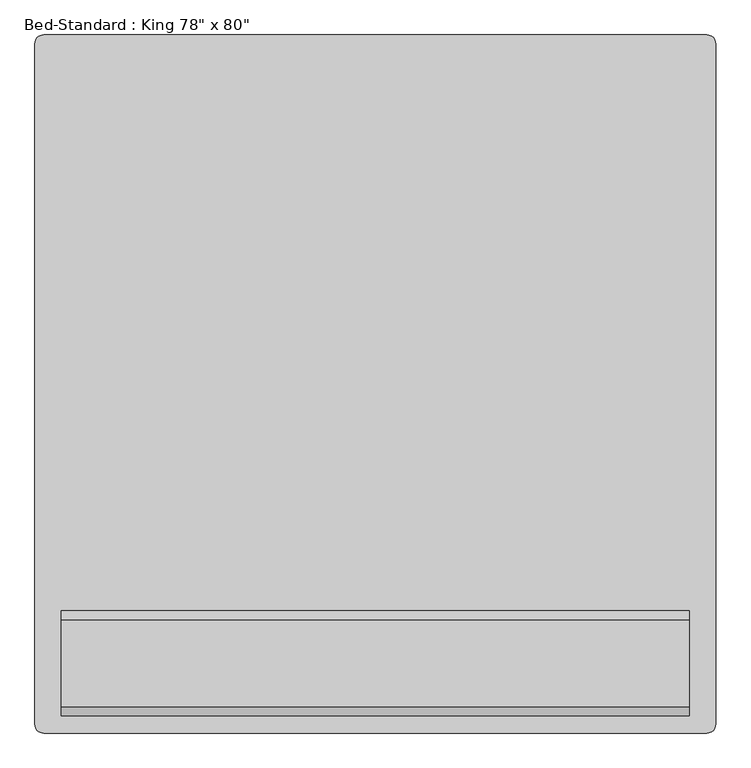
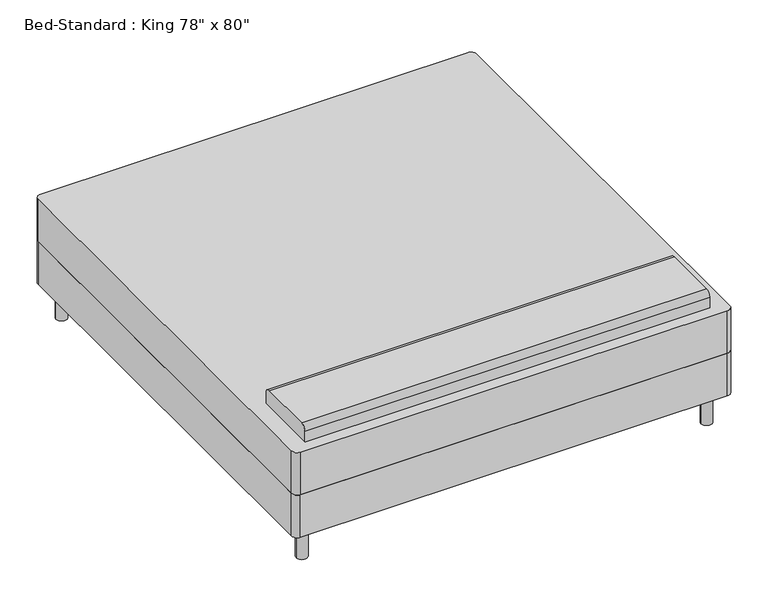
"""IFC4 building model written with IfcOpenShell, lengths in millimetres: furniture geometry."""

from ifc_helpers import new_model, si_unit, point, frame, frame_2d, origin, origin_with_axes, place, context, project, spatial, polyline, circle_curve, trimmed, segment, composite_curve, outline, extrude, source, transform, mapped, element, save


def furniture_df776289(model_context):
    return source(origin(), model_context, "Body", "SweptSolid", [
        extrude(outline(composite_curve([segment(trimmed(circle_curve(frame_2d((-693.7114754, 1036.195082)), 25.4), [point((-719.1114754, 1036.195082))], [point((-693.7114754, 1061.595082))], False, "CARTESIAN"), True, "CONTINUOUS"), segment(polyline([(-693.7114754, 1061.595082), (1236.6885246, 1061.595082)]), True, "CONTINUOUS"), segment(trimmed(circle_curve(frame_2d((1236.6885246, 1036.195082)), 25.4), [point((1236.6885246, 1061.595082))], [point((1262.0885246, 1036.195082))], False, "CARTESIAN"), True, "CONTINUOUS"), segment(polyline([(1262.0885246, 1036.195082), (1262.0885246, -945.004918)]), True, "CONTINUOUS"), segment(trimmed(circle_curve(frame_2d((1236.6885246, -945.004918)), 25.4), [point((1262.0885246, -945.004918))], [point((1236.6885246, -970.404918))], False, "CARTESIAN"), True, "CONTINUOUS"), segment(polyline([(1236.6885246, -970.404918), (-693.7114754, -970.404918)]), True, "CONTINUOUS"), segment(trimmed(circle_curve(frame_2d((-693.7114754, -945.004918)), 25.4), [point((-693.7114754, -970.404918))], [point((-719.1114754, -945.004918))], False, "CARTESIAN"), True, "CONTINUOUS"), segment(polyline([(-719.1114754, -945.004918), (-719.1114754, 1036.195082)]), True, "CONTINUOUS")], self_intersect=False)), frame((0.0, 0.0, 152.4), z_axis=(0.0, 0.0, 1.0), x_axis=(1.0, 0.0, 0.0)), (0.0, 0.0, 1.0), 203.2),
        extrude(outline(composite_curve([segment(polyline([(-614.804918, 558.8), (-919.604918, 558.8), (-919.604918, 609.6)]), True, "CONTINUOUS"), segment(trimmed(circle_curve(frame_2d((-894.204918, 609.6)), 25.4), [point((-919.604918, 609.6))], [point((-894.204918, 635.0))], False, "CARTESIAN"), True, "CONTINUOUS"), segment(polyline([(-894.204918, 635.0), (-640.204918, 635.0)]), True, "CONTINUOUS"), segment(trimmed(circle_curve(frame_2d((-640.204918, 609.6)), 25.4), [point((-640.204918, 635.0))], [point((-614.804918, 609.6))], False, "CARTESIAN"), True, "CONTINUOUS"), segment(polyline([(-614.804918, 609.6), (-614.804918, 558.8)]), True, "CONTINUOUS")], self_intersect=False)), frame((-642.9114754, 0.0, 0.0), z_axis=(1.0, 0.0, 0.0), x_axis=(0.0, 1.0, 0.0)), (0.0, 0.0, 1.0), 1828.8),
        extrude(outline(composite_curve([segment(trimmed(circle_curve(frame_2d((-642.9114754, -894.204918)), 25.4), [point((-668.3114754, -894.204918))], [point((-617.5114754, -894.204918))], False, "CARTESIAN"), True, "CONTINUOUS"), segment(trimmed(circle_curve(frame_2d((-642.9114754, -894.204918)), 25.4), [point((-617.5114754, -894.204918))], [point((-668.3114754, -894.204918))], False, "CARTESIAN"), True, "CONTINUOUS")], self_intersect=False)), origin_with_axes(), (0.0, 0.0, 1.0), 152.4),
        extrude(outline(composite_curve([segment(trimmed(circle_curve(frame_2d((1185.8885246, -894.204918)), 25.4), [point((1160.4885246, -894.204918))], [point((1211.2885246, -894.204918))], False, "CARTESIAN"), True, "CONTINUOUS"), segment(trimmed(circle_curve(frame_2d((1185.8885246, -894.204918)), 25.4), [point((1211.2885246, -894.204918))], [point((1160.4885246, -894.204918))], False, "CARTESIAN"), True, "CONTINUOUS")], self_intersect=False)), origin_with_axes(), (0.0, 0.0, 1.0), 152.4),
        extrude(outline(composite_curve([segment(trimmed(circle_curve(frame_2d((1185.8885246, 985.395082)), 25.4), [point((1160.4885246, 985.395082))], [point((1211.2885246, 985.395082))], False, "CARTESIAN"), True, "CONTINUOUS"), segment(trimmed(circle_curve(frame_2d((1185.8885246, 985.395082)), 25.4), [point((1211.2885246, 985.395082))], [point((1160.4885246, 985.395082))], False, "CARTESIAN"), True, "CONTINUOUS")], self_intersect=False)), origin_with_axes(), (0.0, 0.0, 1.0), 152.4),
        extrude(outline(composite_curve([segment(trimmed(circle_curve(frame_2d((-642.9114754, 985.395082)), 25.4), [point((-668.3114754, 985.395082))], [point((-617.5114754, 985.395082))], False, "CARTESIAN"), True, "CONTINUOUS"), segment(trimmed(circle_curve(frame_2d((-642.9114754, 985.395082)), 25.4), [point((-617.5114754, 985.395082))], [point((-668.3114754, 985.395082))], False, "CARTESIAN"), True, "CONTINUOUS")], self_intersect=False)), origin_with_axes(), (0.0, 0.0, 1.0), 152.4),
        extrude(outline(composite_curve([segment(trimmed(circle_curve(frame_2d((-693.7114754, -945.004918)), 25.4), [point((-693.7114754, -970.404918))], [point((-719.1114754, -945.004918))], False, "CARTESIAN"), True, "CONTINUOUS"), segment(polyline([(-719.1114754, -945.004918), (-719.1114754, 1036.195082)]), True, "CONTINUOUS"), segment(trimmed(circle_curve(frame_2d((-693.7114754, 1036.195082)), 25.4), [point((-719.1114754, 1036.195082))], [point((-693.7114754, 1061.595082))], False, "CARTESIAN"), True, "CONTINUOUS"), segment(polyline([(-693.7114754, 1061.595082), (1236.6885246, 1061.595082)]), True, "CONTINUOUS"), segment(trimmed(circle_curve(frame_2d((1236.6885246, 1036.195082)), 25.4), [point((1236.6885246, 1061.595082))], [point((1262.0885246, 1036.195082))], False, "CARTESIAN"), True, "CONTINUOUS"), segment(polyline([(1262.0885246, 1036.195082), (1262.0885246, -945.004918)]), True, "CONTINUOUS"), segment(trimmed(circle_curve(frame_2d((1236.6885246, -945.004918)), 25.4), [point((1262.0885246, -945.004918))], [point((1236.6885246, -970.404918))], False, "CARTESIAN"), True, "CONTINUOUS"), segment(polyline([(1236.6885246, -970.404918), (-693.7114754, -970.404918)]), True, "CONTINUOUS")], self_intersect=False)), frame((0.0, 0.0, 355.6), z_axis=(0.0, 0.0, 1.0), x_axis=(1.0, 0.0, 0.0)), (0.0, 0.0, 1.0), 203.2),
    ])


if __name__ == "__main__":
    model = new_model("IFC4")
    model_context = context("Model", 3, world=origin())
    ifc_project = project(units=[si_unit("LENGTHUNIT", "METRE", prefix="MILLI")], contexts=[model_context])
    site = spatial("IfcSite", under=ifc_project)
    building = spatial("IfcBuilding", under=site)
    placement = place(None, origin())
    furniture_shape = furniture_df776289(model_context)
    element("IfcFurniture", 1, ObjectType="Bed-Standard : King 78\" x 80\"", at=placement, inside=building, context=model_context, shape_type="MappedRepresentation", body=[
        mapped(furniture_shape, transform((0.0, 0.0, 0.0), x_axis=(1.0, 0.0, 0.0), y_axis=(0.0, 1.0, 0.0), z_axis=(0.0, 0.0, 1.0))),
    ])
    save(model, "model.ifc")

# Revit data of these elements
# Type "Bed-Standard : King 78\" x 80\""
#   Assembly Code = "E2020200"
#   Clear Dim_2 = 2' - 0"
#   Clear Dim_1 = 3' - 0"
#   Length = 6' - 8"
#   Width = 6' - 6"
#   Leg Material = Metal - Chrome
#   Mattress Material = Textile - White
# Element 1 (IfcFurniture, "Bed-Standard : King 78\" x 80\"")
#   Materials on its faces: "Textile - White", "Metal - Chrome"
# Materials
#   "Metal - Chrome": class "Metal", colour RGB 17 17 17, transparency 0
#   "Textile - White": class "Fabric", colour RGB 247 247 239, transparency 0
